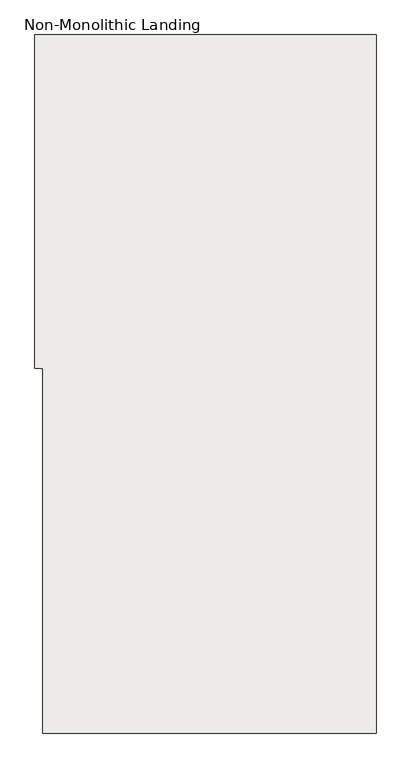
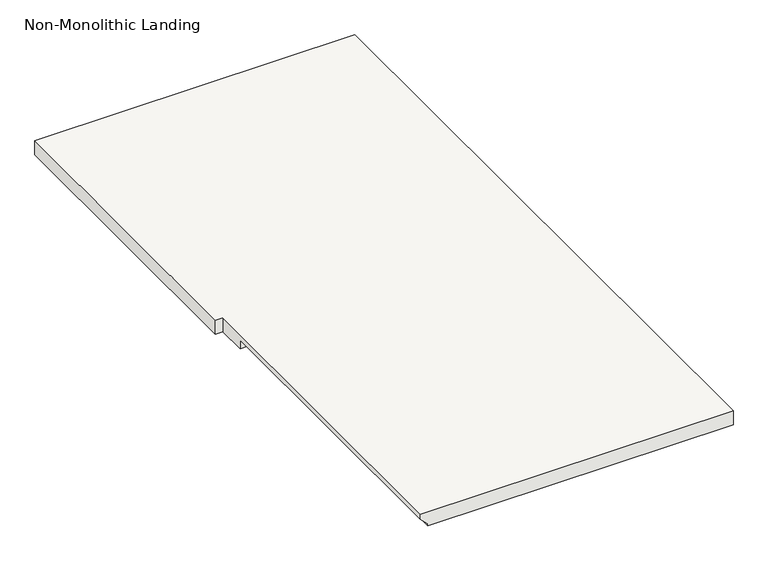
"""IFC4 building model written with IfcOpenShell, lengths in millimetres: slab geometry, Non-Monolithic Landing."""

import ifcopenshell
import ifcopenshell.guid

model = None  # the IFC model being written
_history = None  # IfcOwnerHistory: only IFC2X3 demands one
_inside = {}  # id of a spatial element -> (the spatial element, [elements in it])
_under = {}  # id of a project, library or spatial element -> (it, [spatial elements below it])
_declared = {}  # id of a project -> (the project, [libraries it declares])
_typed = {}  # id of a type object -> (the type object, [elements of that type])
_made_of = {}  # id of a material, layer set ... -> (it, [elements and type objects made of it])


def new_model(schema):
    """Start an empty IFC model of exactly this schema.

    Asked for "IFC4X3", IfcOpenShell would pick the latest addendum, in which some entities
    have other attributes; the version numbers below select the first issue.
    IFC2X3 requires an IfcOwnerHistory on every rooted entity: one is made here for all.
    """
    global model, _history
    if schema == "IFC4X3":
        model = ifcopenshell.file(schema_version=(4, 3, 0, 0))
    else:
        model = ifcopenshell.file(schema=schema)
    _inside.clear()
    _under.clear()
    _declared.clear()
    _typed.clear()
    _made_of.clear()
    _history = None
    if model.schema == "IFC2X3":
        org = make("IfcOrganization", Name="unknown")
        user = make(
            "IfcPersonAndOrganization",
            ThePerson=make("IfcPerson", FamilyName="unknown"),
            TheOrganization=org,
        )
        app = make(
            "IfcApplication",
            ApplicationDeveloper=org,
            Version="unknown",
            ApplicationFullName="unknown",
            ApplicationIdentifier="unknown",
        )
        _history = make(
            "IfcOwnerHistory",
            OwningUser=user,
            OwningApplication=app,
            ChangeAction="ADDED",
            CreationDate=0,
        )
    return model


def make(cls, **values):
    """One entity of the class cls with the attributes given. An attribute that is None is left unset."""
    return model.create_entity(
        cls, **{name: value for name, value in values.items() if value is not None}
    )


def rooted(cls, **values):
    """An entity with a GlobalId (a new one), such as an element, a storey or a relation."""
    return make(cls, GlobalId=ifcopenshell.guid.new(), OwnerHistory=_history, **values)


def si_unit(unit_type, name, prefix=None):
    """IfcSIUnit, for example si_unit("LENGTHUNIT", "METRE", prefix="MILLI")."""
    return make("IfcSIUnit", UnitType=unit_type, Prefix=prefix, Name=name)


def assignment(units):
    """IfcUnitAssignment: the units of a project."""
    return None if units is None else make("IfcUnitAssignment", Units=units)


def point(xyz):
    """IfcCartesianPoint."""
    return None if xyz is None else make("IfcCartesianPoint", Coordinates=xyz)


def direction(xyz):
    """IfcDirection."""
    return None if xyz is None else make("IfcDirection", DirectionRatios=xyz)


def frame(location, z_axis=None, x_axis=None):
    """IfcAxis2Placement3D, a coordinate frame: its origin and axes. An axis left out is left unset."""
    return make(
        "IfcAxis2Placement3D",
        Location=point(location),
        Axis=direction(z_axis),
        RefDirection=direction(x_axis),
    )


def origin():
    """The frame at (0, 0, 0) with its axes left unset."""
    return frame((0.0, 0.0, 0.0))


def place(relative_to, where):
    """IfcLocalPlacement: puts the frame where relative to a parent placement (None: the world)."""
    return make(
        "IfcLocalPlacement", PlacementRelTo=relative_to, RelativePlacement=where
    )


def context(
    kind, dimensions, precision=None, world=None, true_north=None, identifier=None
):
    """IfcGeometricRepresentationContext, for example the 3D "Model" context."""
    return make(
        "IfcGeometricRepresentationContext",
        ContextIdentifier=identifier,
        ContextType=kind,
        CoordinateSpaceDimension=dimensions,
        Precision=precision,
        WorldCoordinateSystem=world,
        TrueNorth=true_north,
    )


def project(units=None, contexts=None):
    """IfcProject with its units and contexts."""
    return rooted(
        "IfcProject",
        Name="project",
        RepresentationContexts=contexts,
        UnitsInContext=assignment(units),
    )


def spatial(cls, under=None, at=None, **own):
    """A site, building, storey or space (cls), placed at a placement, below another one or the project."""
    s = rooted(cls, ObjectPlacement=at, **own)
    if under is not None:
        _under.setdefault(under.id(), (under, []))[1].append(s)
    return s


def faces_of(points, faces, orient=None, outer=None):
    """IfcFace entities. A face is a list of loops; a loop is a list of indices into points, from 0.

    orient and outer hold one flag for each loop. By default every Orientation is true, the
    first loop of a face is its IfcFaceOuterBound and the others are IfcFaceBound.
    """
    made = []
    for i, loops in enumerate(faces):
        bounds = []
        for j, loop in enumerate(loops):
            is_outer = j == 0 if outer is None else outer[i][j]
            bounds.append(
                make(
                    "IfcFaceOuterBound" if is_outer else "IfcFaceBound",
                    Bound=make("IfcPolyLoop", Polygon=[points[k] for k in loop]),
                    Orientation=True if orient is None else orient[i][j],
                )
            )
        made.append(make("IfcFace", Bounds=bounds))
    return made


def faceted_brep(points, faces, orient=None, outer=None, voids=None):
    """IfcFacetedBrep: a solid bounded by flat faces; with voids (closed shells), ...WithVoids."""
    shared = [point(p) for p in points]
    hull = make("IfcClosedShell", CfsFaces=faces_of(shared, faces, orient, outer))
    if voids is None:
        return make("IfcFacetedBrep", Outer=hull)
    return make(
        "IfcFacetedBrepWithVoids",
        Outer=hull,
        Voids=[
            make(cls, CfsFaces=faces_of(shared, fs, o, b)) for cls, fs, o, b in voids
        ],
    )


def shape(context_of_items, identifier, shape_type, items):
    """IfcShapeRepresentation: the items that make up one representation, for example the "Body"."""
    return make(
        "IfcShapeRepresentation",
        ContextOfItems=context_of_items,
        RepresentationIdentifier=identifier,
        RepresentationType=shape_type,
        Items=items,
    )


def source(mapping_origin, context_of_items, identifier, shape_type, items):
    """IfcRepresentationMap: a shape defined once, which mapped items show again and again."""
    return make(
        "IfcRepresentationMap",
        MappingOrigin=mapping_origin,
        MappedRepresentation=shape(context_of_items, identifier, shape_type, items),
    )


def transform(
    local_origin,
    x_axis=None,
    y_axis=None,
    z_axis=None,
    scale=None,
    scale2=None,
    scale3=None,
    uniform=True,
):
    """IfcCartesianTransformationOperator3D, or its non-uniform kind. x_axis, y_axis, z_axis: its Axis1, 2, 3."""
    if uniform:
        return make(
            "IfcCartesianTransformationOperator3D",
            Axis1=direction(x_axis),
            Axis2=direction(y_axis),
            LocalOrigin=point(local_origin),
            Scale=scale,
            Axis3=direction(z_axis),
        )
    return make(
        "IfcCartesianTransformationOperator3DnonUniform",
        Axis1=direction(x_axis),
        Axis2=direction(y_axis),
        LocalOrigin=point(local_origin),
        Scale=scale,
        Axis3=direction(z_axis),
        Scale2=scale2,
        Scale3=scale3,
    )


def mapped(mapping_source, mapping_target):
    """IfcMappedItem: shows the shape of a source again, moved by a transform."""
    return make(
        "IfcMappedItem", MappingSource=mapping_source, MappingTarget=mapping_target
    )


def made_of(thing, what):
    """Note that an element or type object is made of a material, layer set ...; save() writes the relation."""
    if what is not None:
        _made_of.setdefault(what.id(), (what, []))[1].append(thing)
    return thing


def element(
    cls,
    number,
    at=None,
    inside=None,
    cuts=None,
    type_object=None,
    material=None,
    context=None,
    identifier="Body",
    shape_type=None,
    held_by="IfcProductDefinitionShape",
    body=None,
    shapes=None,
    **own,
):
    """One element of the class cls, such as IfcWall. Its Tag is "e" and its number.

    at: its placement. inside: the storey or other place that contains it. cuts: it is an
    opening in that element (IfcRelVoidsElement). A single representation is given by context,
    identifier, shape_type and body (its items); several are given by shapes. held_by: the class
    of the entity that holds the representations. save() writes the other relations.
    """
    e = rooted(cls, Tag="e%d" % number, ObjectPlacement=at, **own)
    if body is not None:
        shapes = [shape(context, identifier, shape_type, body)]
    if shapes is not None:
        e.Representation = make(held_by, Representations=shapes)
    if inside is not None:
        _inside.setdefault(inside.id(), (inside, []))[1].append(e)
    if cuts is not None:
        rooted(
            "IfcRelVoidsElement", RelatingBuildingElement=cuts, RelatedOpeningElement=e
        )
    if type_object is not None:
        _typed.setdefault(type_object.id(), (type_object, []))[1].append(e)
    return made_of(e, material)


def aggregate(whole, parts):
    """IfcRelAggregates: a whole, such as a stair, and the parts it consists of."""
    return rooted("IfcRelAggregates", RelatingObject=whole, RelatedObjects=parts)


def save(model, path):
    """Write the relations noted so far, then the file.

    IfcRelAggregates (storeys below a building ...), IfcRelContainedInSpatialStructure (elements
    in a storey), IfcRelDefinesByType, IfcRelAssociatesMaterial and IfcRelDeclares: one each for
    every whole, place, type object, material and project.
    """
    for whole, parts in _under.values():
        aggregate(whole, parts)
    for where, things in _inside.values():
        rooted(
            "IfcRelContainedInSpatialStructure",
            RelatedElements=things,
            RelatingStructure=where,
        )
    for kind, things in _typed.values():
        rooted("IfcRelDefinesByType", RelatedObjects=things, RelatingType=kind)
    for what, things in _made_of.values():
        rooted("IfcRelAssociatesMaterial", RelatedObjects=things, RelatingMaterial=what)
    for by, libraries in _declared.values():
        rooted("IfcRelDeclares", RelatingContext=by, RelatedDefinitions=libraries)
    model.write(path)


def non_monolithic_landing_e50ec3fc(model_context):
    return source(origin(), model_context, "Body", "Brep", [
        faceted_brep([(665981.788677, -551651.2413841, 4737.6148649), (665956.388677, -551651.2413841, 4763.0148649), (665956.388677, -550584.4413841, 4763.0148649), (665981.788677, -550584.4413841, 4737.6148649), (667023.188677, -551651.2413841, 4782.0648649), (667023.188677, -549416.0413841, 4782.0648649), (665956.388677, -549416.0413841, 4782.0648649), (665930.988677, -549416.0413841, 4782.0648649), (665930.988677, -550482.8413841, 4782.0648649), (665956.388677, -550482.8413841, 4782.0648649), (665956.388677, -551651.2413841, 4782.0648649), (665981.788677, -550584.4413841, 4731.2648649), (665956.388677, -550584.4413841, 4731.2648649), (665956.388677, -550482.8413841, 4731.2648649), (665930.988677, -550482.8413841, 4731.2648649), (665930.988677, -549416.0413841, 4731.2648649), (665956.388677, -549416.0413841, 4731.2648649), (667023.188677, -549416.0413841, 4731.2648649), (667023.188677, -551651.2413841, 4731.2648649), (665981.788677, -551651.2413841, 4731.2648649)], [[[0, 1, 2, 3]], [[4, 5, 6, 7, 8, 9, 10]], [[11, 12, 13, 14, 15, 16, 17, 18, 19]], [[12, 11, 3, 2]], [[11, 19, 0, 3]], [[4, 10, 1, 0, 19, 18]], [[5, 4, 18, 17]], [[6, 5, 17, 16]], [[7, 6, 16, 15]], [[8, 7, 15, 14]], [[9, 8, 14, 13]], [[10, 9, 13, 12, 2, 1]]]),
    ])


if __name__ == "__main__":
    model = new_model("IFC4")
    model_context = context("Model", 3, world=origin())
    ifc_project = project(units=[si_unit("LENGTHUNIT", "METRE", prefix="MILLI")], contexts=[model_context])
    site = spatial("IfcSite", under=ifc_project)
    building = spatial("IfcBuilding", under=site)
    placement = place(None, origin())
    non_monolithic_landing_shape = non_monolithic_landing_e50ec3fc(model_context)
    element("IfcSlab", 1, ObjectType="Non-Monolithic Landing", at=placement, inside=building, context=model_context, shape_type="MappedRepresentation", body=[
        mapped(non_monolithic_landing_shape, transform((0.0, 0.0, 0.0), x_axis=(1.0, 0.0, 0.0), y_axis=(0.0, 1.0, 0.0), z_axis=(0.0, 0.0, 1.0))),
    ])
    save(model, "model.ifc")
